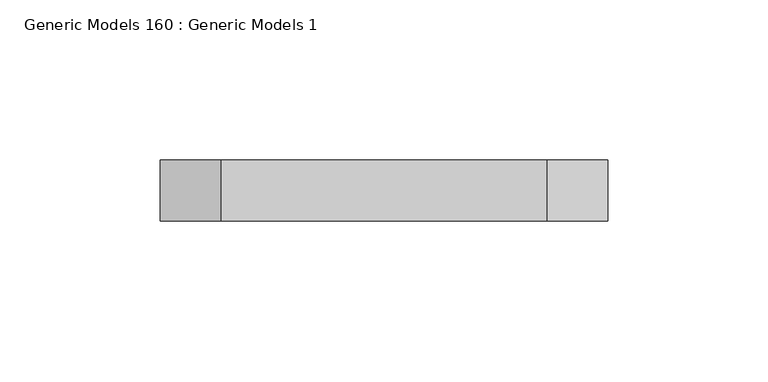
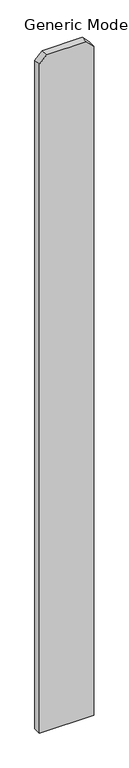
"""IFC4 building model written with IfcOpenShell, lengths in millimetres: proxy geometry, Generic Models 160 : Generic Models 1."""

import ifcopenshell
import ifcopenshell.guid

model = None  # the IFC model being written
_history = None  # IfcOwnerHistory: only IFC2X3 demands one
_inside = {}  # id of a spatial element -> (the spatial element, [elements in it])
_under = {}  # id of a project, library or spatial element -> (it, [spatial elements below it])
_declared = {}  # id of a project -> (the project, [libraries it declares])
_typed = {}  # id of a type object -> (the type object, [elements of that type])
_made_of = {}  # id of a material, layer set ... -> (it, [elements and type objects made of it])


def new_model(schema):
    """Start an empty IFC model of exactly this schema.

    Asked for "IFC4X3", IfcOpenShell would pick the latest addendum, in which some entities
    have other attributes; the version numbers below select the first issue.
    IFC2X3 requires an IfcOwnerHistory on every rooted entity: one is made here for all.
    """
    global model, _history
    if schema == "IFC4X3":
        model = ifcopenshell.file(schema_version=(4, 3, 0, 0))
    else:
        model = ifcopenshell.file(schema=schema)
    _inside.clear()
    _under.clear()
    _declared.clear()
    _typed.clear()
    _made_of.clear()
    _history = None
    if model.schema == "IFC2X3":
        org = make("IfcOrganization", Name="unknown")
        user = make(
            "IfcPersonAndOrganization",
            ThePerson=make("IfcPerson", FamilyName="unknown"),
            TheOrganization=org,
        )
        app = make(
            "IfcApplication",
            ApplicationDeveloper=org,
            Version="unknown",
            ApplicationFullName="unknown",
            ApplicationIdentifier="unknown",
        )
        _history = make(
            "IfcOwnerHistory",
            OwningUser=user,
            OwningApplication=app,
            ChangeAction="ADDED",
            CreationDate=0,
        )
    return model


def make(cls, **values):
    """One entity of the class cls with the attributes given. An attribute that is None is left unset."""
    return model.create_entity(
        cls, **{name: value for name, value in values.items() if value is not None}
    )


def rooted(cls, **values):
    """An entity with a GlobalId (a new one), such as an element, a storey or a relation."""
    return make(cls, GlobalId=ifcopenshell.guid.new(), OwnerHistory=_history, **values)


def si_unit(unit_type, name, prefix=None):
    """IfcSIUnit, for example si_unit("LENGTHUNIT", "METRE", prefix="MILLI")."""
    return make("IfcSIUnit", UnitType=unit_type, Prefix=prefix, Name=name)


def assignment(units):
    """IfcUnitAssignment: the units of a project."""
    return None if units is None else make("IfcUnitAssignment", Units=units)


def point(xyz):
    """IfcCartesianPoint."""
    return None if xyz is None else make("IfcCartesianPoint", Coordinates=xyz)


def direction(xyz):
    """IfcDirection."""
    return None if xyz is None else make("IfcDirection", DirectionRatios=xyz)


def frame(location, z_axis=None, x_axis=None):
    """IfcAxis2Placement3D, a coordinate frame: its origin and axes. An axis left out is left unset."""
    return make(
        "IfcAxis2Placement3D",
        Location=point(location),
        Axis=direction(z_axis),
        RefDirection=direction(x_axis),
    )


def origin():
    """The frame at (0, 0, 0) with its axes left unset."""
    return frame((0.0, 0.0, 0.0))


def place(relative_to, where):
    """IfcLocalPlacement: puts the frame where relative to a parent placement (None: the world)."""
    return make(
        "IfcLocalPlacement", PlacementRelTo=relative_to, RelativePlacement=where
    )


def context(
    kind, dimensions, precision=None, world=None, true_north=None, identifier=None
):
    """IfcGeometricRepresentationContext, for example the 3D "Model" context."""
    return make(
        "IfcGeometricRepresentationContext",
        ContextIdentifier=identifier,
        ContextType=kind,
        CoordinateSpaceDimension=dimensions,
        Precision=precision,
        WorldCoordinateSystem=world,
        TrueNorth=true_north,
    )


def project(units=None, contexts=None):
    """IfcProject with its units and contexts."""
    return rooted(
        "IfcProject",
        Name="project",
        RepresentationContexts=contexts,
        UnitsInContext=assignment(units),
    )


def spatial(cls, under=None, at=None, **own):
    """A site, building, storey or space (cls), placed at a placement, below another one or the project."""
    s = rooted(cls, ObjectPlacement=at, **own)
    if under is not None:
        _under.setdefault(under.id(), (under, []))[1].append(s)
    return s


def polyline(points):
    """IfcPolyline through the points."""
    return make("IfcPolyline", Points=[point(p) for p in points])


def outline(outer, holes=None, kind="AREA"):
    """IfcArbitraryClosedProfileDef: a profile drawn as a closed curve; with holes, ...WithVoids."""
    if holes is None:
        return make("IfcArbitraryClosedProfileDef", ProfileType=kind, OuterCurve=outer)
    return make(
        "IfcArbitraryProfileDefWithVoids",
        ProfileType=kind,
        OuterCurve=outer,
        InnerCurves=holes,
    )


def extrude(swept, where, along, depth):
    """IfcExtrudedAreaSolid: the profile swept, set in the frame where, extruded along a direction by depth."""
    return make(
        "IfcExtrudedAreaSolid",
        SweptArea=swept,
        Position=where,
        ExtrudedDirection=direction(along),
        Depth=depth,
    )


def shape(context_of_items, identifier, shape_type, items):
    """IfcShapeRepresentation: the items that make up one representation, for example the "Body"."""
    return make(
        "IfcShapeRepresentation",
        ContextOfItems=context_of_items,
        RepresentationIdentifier=identifier,
        RepresentationType=shape_type,
        Items=items,
    )


def source(mapping_origin, context_of_items, identifier, shape_type, items):
    """IfcRepresentationMap: a shape defined once, which mapped items show again and again."""
    return make(
        "IfcRepresentationMap",
        MappingOrigin=mapping_origin,
        MappedRepresentation=shape(context_of_items, identifier, shape_type, items),
    )


def transform(
    local_origin,
    x_axis=None,
    y_axis=None,
    z_axis=None,
    scale=None,
    scale2=None,
    scale3=None,
    uniform=True,
):
    """IfcCartesianTransformationOperator3D, or its non-uniform kind. x_axis, y_axis, z_axis: its Axis1, 2, 3."""
    if uniform:
        return make(
            "IfcCartesianTransformationOperator3D",
            Axis1=direction(x_axis),
            Axis2=direction(y_axis),
            LocalOrigin=point(local_origin),
            Scale=scale,
            Axis3=direction(z_axis),
        )
    return make(
        "IfcCartesianTransformationOperator3DnonUniform",
        Axis1=direction(x_axis),
        Axis2=direction(y_axis),
        LocalOrigin=point(local_origin),
        Scale=scale,
        Axis3=direction(z_axis),
        Scale2=scale2,
        Scale3=scale3,
    )


def mapped(mapping_source, mapping_target):
    """IfcMappedItem: shows the shape of a source again, moved by a transform."""
    return make(
        "IfcMappedItem", MappingSource=mapping_source, MappingTarget=mapping_target
    )


def made_of(thing, what):
    """Note that an element or type object is made of a material, layer set ...; save() writes the relation."""
    if what is not None:
        _made_of.setdefault(what.id(), (what, []))[1].append(thing)
    return thing


def element(
    cls,
    number,
    at=None,
    inside=None,
    cuts=None,
    type_object=None,
    material=None,
    context=None,
    identifier="Body",
    shape_type=None,
    held_by="IfcProductDefinitionShape",
    body=None,
    shapes=None,
    **own,
):
    """One element of the class cls, such as IfcWall. Its Tag is "e" and its number.

    at: its placement. inside: the storey or other place that contains it. cuts: it is an
    opening in that element (IfcRelVoidsElement). A single representation is given by context,
    identifier, shape_type and body (its items); several are given by shapes. held_by: the class
    of the entity that holds the representations. save() writes the other relations.
    """
    e = rooted(cls, Tag="e%d" % number, ObjectPlacement=at, **own)
    if body is not None:
        shapes = [shape(context, identifier, shape_type, body)]
    if shapes is not None:
        e.Representation = make(held_by, Representations=shapes)
    if inside is not None:
        _inside.setdefault(inside.id(), (inside, []))[1].append(e)
    if cuts is not None:
        rooted(
            "IfcRelVoidsElement", RelatingBuildingElement=cuts, RelatedOpeningElement=e
        )
    if type_object is not None:
        _typed.setdefault(type_object.id(), (type_object, []))[1].append(e)
    return made_of(e, material)


def aggregate(whole, parts):
    """IfcRelAggregates: a whole, such as a stair, and the parts it consists of."""
    return rooted("IfcRelAggregates", RelatingObject=whole, RelatedObjects=parts)


def save(model, path):
    """Write the relations noted so far, then the file.

    IfcRelAggregates (storeys below a building ...), IfcRelContainedInSpatialStructure (elements
    in a storey), IfcRelDefinesByType, IfcRelAssociatesMaterial and IfcRelDeclares: one each for
    every whole, place, type object, material and project.
    """
    for whole, parts in _under.values():
        aggregate(whole, parts)
    for where, things in _inside.values():
        rooted(
            "IfcRelContainedInSpatialStructure",
            RelatedElements=things,
            RelatingStructure=where,
        )
    for kind, things in _typed.values():
        rooted("IfcRelDefinesByType", RelatedObjects=things, RelatingType=kind)
    for what, things in _made_of.values():
        rooted("IfcRelAssociatesMaterial", RelatedObjects=things, RelatingMaterial=what)
    for by, libraries in _declared.values():
        rooted("IfcRelDeclares", RelatingContext=by, RelatedDefinitions=libraries)
    model.write(path)


def generic_models_160_generic_models_1_9801a194(model_context):
    return source(origin(), model_context, "Body", "SweptSolid", [
        extrude(outline(polyline([(76.2, 54379.8125), (1885.95, 54379.8125), (1905.0, 54360.7625), (1905.0, 54259.1625), (1885.95, 54240.1125), (76.2, 54240.1125), (76.2, 54379.8125)])), frame((0.0, 547.6875, 0.0), z_axis=(0.0, 1.0, 0.0), x_axis=(0.0, 0.0, 1.0)), (0.0, 0.0, 1.0), 19.05),
    ])


if __name__ == "__main__":
    model = new_model("IFC4")
    model_context = context("Model", 3, world=origin())
    ifc_project = project(units=[si_unit("LENGTHUNIT", "METRE", prefix="MILLI")], contexts=[model_context])
    site = spatial("IfcSite", under=ifc_project)
    building = spatial("IfcBuilding", under=site)
    placement = place(None, origin())
    generic_models_160_generic_models_1_shape = generic_models_160_generic_models_1_9801a194(model_context)
    element("IfcBuildingElementProxy", 1, Name="Generic Models 160 : Generic Models 1", ObjectType="Generic Models 160 : Generic Models 1", at=placement, inside=building, context=model_context, shape_type="MappedRepresentation", body=[
        mapped(generic_models_160_generic_models_1_shape, transform((0.0, 0.0, 0.0), x_axis=(1.0, 0.0, 0.0), y_axis=(0.0, 1.0, 0.0), z_axis=(0.0, 0.0, 1.0))),
    ])
    save(model, "model.ifc")

# Revit data of these elements
# Element 1 (IfcBuildingElementProxy, "Generic Models 160 : Generic Models 1")
#   Materials on its faces: "VERTICAL 1X6 CEDAR PLANKS W/ CLEAR WOOD SEALER"
# Materials
#   "VERTICAL 1X6 CEDAR PLANKS W/ CLEAR WOOD SEALER": class "Wood", colour RGB 234 198 147, transparency 0, Description = "Pinus Echinata", Cost = 0
